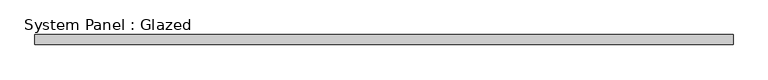
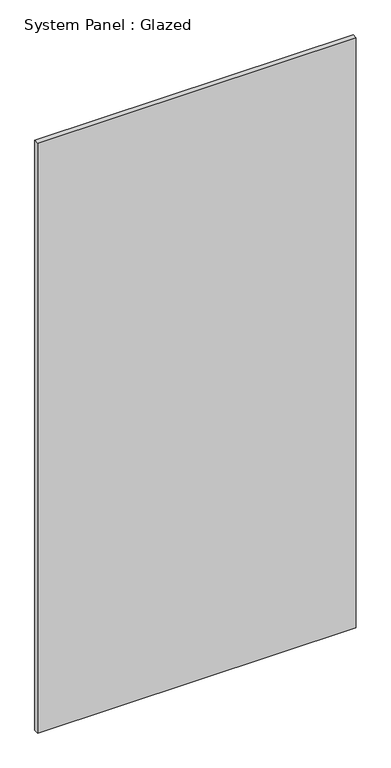
"""IFC4 building model written with IfcOpenShell, lengths in millimetres: plate geometry, System Panel : Glazed."""

from ifc_helpers import new_model, si_unit, origin, origin_with_axes, place, context, project, spatial, polyline, outline, extrude, source, transform, mapped, element, save


def system_panel_glazed_6c0831e3(model_context):
    return source(origin(), model_context, "Body", "SweptSolid", [
        extrude(outline(polyline([(882.65, 19.05), (-882.65, 19.05), (-882.65, 44.45), (882.65, 44.45), (882.65, 19.05)])), origin_with_axes(), (0.0, 0.0, 1.0), 3454.4),
    ])


if __name__ == "__main__":
    model = new_model("IFC4")
    model_context = context("Model", 3, world=origin())
    ifc_project = project(units=[si_unit("LENGTHUNIT", "METRE", prefix="MILLI")], contexts=[model_context])
    site = spatial("IfcSite", under=ifc_project)
    building = spatial("IfcBuilding", under=site)
    placement = place(None, origin())
    system_panel_glazed_shape = system_panel_glazed_6c0831e3(model_context)
    element("IfcPlate", 1, ObjectType="System Panel : Glazed", at=placement, inside=building, context=model_context, shape_type="MappedRepresentation", body=[
        mapped(system_panel_glazed_shape, transform((0.0, 0.0, 0.0), x_axis=(1.0, 0.0, 0.0), y_axis=(0.0, 1.0, 0.0), z_axis=(0.0, 0.0, 1.0))),
    ])
    save(model, "model.ifc")

# Revit data of these elements
# Type "System Panel : Glazed"
#   Construction Type Id = "GSP4R"
#   Analytic Construction = "1/8 in Pilkington single glazing"
#   Visual Light Transmittance = 0.9
#   Solar Heat Gain Coefficient = 0.86
#   Heat Transfer Coefficient (U) = 1.18115 BTU/(h·ft²·°F)
#   Define Thermal Properties by = 1
# Element 1 (IfcPlate, "System Panel : Glazed")
#   Materials on its faces: "Glass"
# Materials
#   "Glass": class "Glass", colour RGB 0 128 192, transparency 0.75, Description = "Soda Lime Glass", Cost = 0
